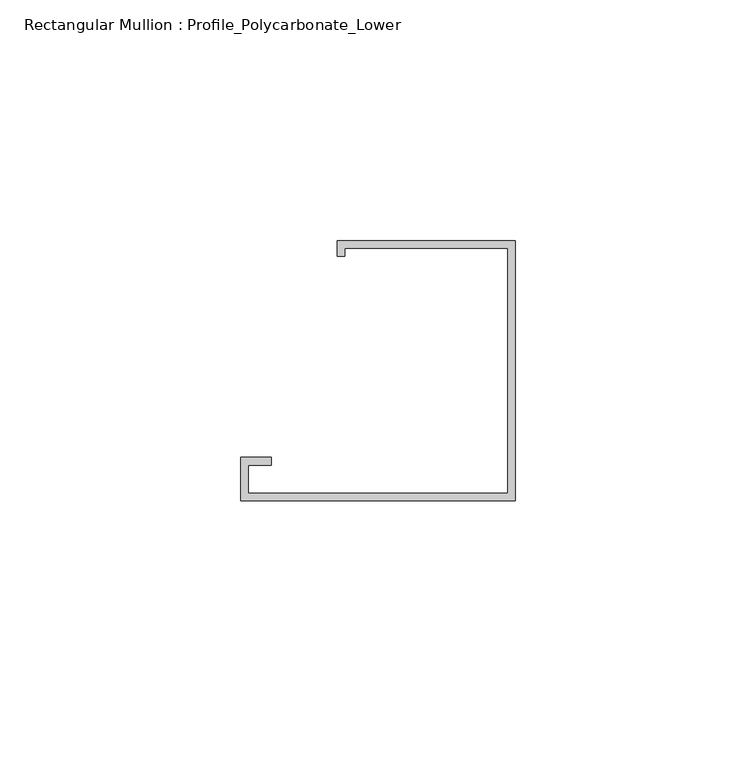
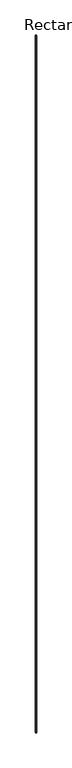
"""IFC4 building model written with IfcOpenShell, lengths in millimetres: member geometry, Rectangular Mullion : Profile_Polycarbonate_Lower."""

import ifcopenshell
import ifcopenshell.guid

model = None  # the IFC model being written
_history = None  # IfcOwnerHistory: only IFC2X3 demands one
_inside = {}  # id of a spatial element -> (the spatial element, [elements in it])
_under = {}  # id of a project, library or spatial element -> (it, [spatial elements below it])
_declared = {}  # id of a project -> (the project, [libraries it declares])
_typed = {}  # id of a type object -> (the type object, [elements of that type])
_made_of = {}  # id of a material, layer set ... -> (it, [elements and type objects made of it])


def new_model(schema):
    """Start an empty IFC model of exactly this schema.

    Asked for "IFC4X3", IfcOpenShell would pick the latest addendum, in which some entities
    have other attributes; the version numbers below select the first issue.
    IFC2X3 requires an IfcOwnerHistory on every rooted entity: one is made here for all.
    """
    global model, _history
    if schema == "IFC4X3":
        model = ifcopenshell.file(schema_version=(4, 3, 0, 0))
    else:
        model = ifcopenshell.file(schema=schema)
    _inside.clear()
    _under.clear()
    _declared.clear()
    _typed.clear()
    _made_of.clear()
    _history = None
    if model.schema == "IFC2X3":
        org = make("IfcOrganization", Name="unknown")
        user = make(
            "IfcPersonAndOrganization",
            ThePerson=make("IfcPerson", FamilyName="unknown"),
            TheOrganization=org,
        )
        app = make(
            "IfcApplication",
            ApplicationDeveloper=org,
            Version="unknown",
            ApplicationFullName="unknown",
            ApplicationIdentifier="unknown",
        )
        _history = make(
            "IfcOwnerHistory",
            OwningUser=user,
            OwningApplication=app,
            ChangeAction="ADDED",
            CreationDate=0,
        )
    return model


def make(cls, **values):
    """One entity of the class cls with the attributes given. An attribute that is None is left unset."""
    return model.create_entity(
        cls, **{name: value for name, value in values.items() if value is not None}
    )


def rooted(cls, **values):
    """An entity with a GlobalId (a new one), such as an element, a storey or a relation."""
    return make(cls, GlobalId=ifcopenshell.guid.new(), OwnerHistory=_history, **values)


def si_unit(unit_type, name, prefix=None):
    """IfcSIUnit, for example si_unit("LENGTHUNIT", "METRE", prefix="MILLI")."""
    return make("IfcSIUnit", UnitType=unit_type, Prefix=prefix, Name=name)


def assignment(units):
    """IfcUnitAssignment: the units of a project."""
    return None if units is None else make("IfcUnitAssignment", Units=units)


def point(xyz):
    """IfcCartesianPoint."""
    return None if xyz is None else make("IfcCartesianPoint", Coordinates=xyz)


def direction(xyz):
    """IfcDirection."""
    return None if xyz is None else make("IfcDirection", DirectionRatios=xyz)


def frame(location, z_axis=None, x_axis=None):
    """IfcAxis2Placement3D, a coordinate frame: its origin and axes. An axis left out is left unset."""
    return make(
        "IfcAxis2Placement3D",
        Location=point(location),
        Axis=direction(z_axis),
        RefDirection=direction(x_axis),
    )


def origin():
    """The frame at (0, 0, 0) with its axes left unset."""
    return frame((0.0, 0.0, 0.0))


def place(relative_to, where):
    """IfcLocalPlacement: puts the frame where relative to a parent placement (None: the world)."""
    return make(
        "IfcLocalPlacement", PlacementRelTo=relative_to, RelativePlacement=where
    )


def context(
    kind, dimensions, precision=None, world=None, true_north=None, identifier=None
):
    """IfcGeometricRepresentationContext, for example the 3D "Model" context."""
    return make(
        "IfcGeometricRepresentationContext",
        ContextIdentifier=identifier,
        ContextType=kind,
        CoordinateSpaceDimension=dimensions,
        Precision=precision,
        WorldCoordinateSystem=world,
        TrueNorth=true_north,
    )


def project(units=None, contexts=None):
    """IfcProject with its units and contexts."""
    return rooted(
        "IfcProject",
        Name="project",
        RepresentationContexts=contexts,
        UnitsInContext=assignment(units),
    )


def spatial(cls, under=None, at=None, **own):
    """A site, building, storey or space (cls), placed at a placement, below another one or the project."""
    s = rooted(cls, ObjectPlacement=at, **own)
    if under is not None:
        _under.setdefault(under.id(), (under, []))[1].append(s)
    return s


def polyline(points):
    """IfcPolyline through the points."""
    return make("IfcPolyline", Points=[point(p) for p in points])


def outline(outer, holes=None, kind="AREA"):
    """IfcArbitraryClosedProfileDef: a profile drawn as a closed curve; with holes, ...WithVoids."""
    if holes is None:
        return make("IfcArbitraryClosedProfileDef", ProfileType=kind, OuterCurve=outer)
    return make(
        "IfcArbitraryProfileDefWithVoids",
        ProfileType=kind,
        OuterCurve=outer,
        InnerCurves=holes,
    )


def extrude(swept, where, along, depth):
    """IfcExtrudedAreaSolid: the profile swept, set in the frame where, extruded along a direction by depth."""
    return make(
        "IfcExtrudedAreaSolid",
        SweptArea=swept,
        Position=where,
        ExtrudedDirection=direction(along),
        Depth=depth,
    )


def shape(context_of_items, identifier, shape_type, items):
    """IfcShapeRepresentation: the items that make up one representation, for example the "Body"."""
    return make(
        "IfcShapeRepresentation",
        ContextOfItems=context_of_items,
        RepresentationIdentifier=identifier,
        RepresentationType=shape_type,
        Items=items,
    )


def source(mapping_origin, context_of_items, identifier, shape_type, items):
    """IfcRepresentationMap: a shape defined once, which mapped items show again and again."""
    return make(
        "IfcRepresentationMap",
        MappingOrigin=mapping_origin,
        MappedRepresentation=shape(context_of_items, identifier, shape_type, items),
    )


def transform(
    local_origin,
    x_axis=None,
    y_axis=None,
    z_axis=None,
    scale=None,
    scale2=None,
    scale3=None,
    uniform=True,
):
    """IfcCartesianTransformationOperator3D, or its non-uniform kind. x_axis, y_axis, z_axis: its Axis1, 2, 3."""
    if uniform:
        return make(
            "IfcCartesianTransformationOperator3D",
            Axis1=direction(x_axis),
            Axis2=direction(y_axis),
            LocalOrigin=point(local_origin),
            Scale=scale,
            Axis3=direction(z_axis),
        )
    return make(
        "IfcCartesianTransformationOperator3DnonUniform",
        Axis1=direction(x_axis),
        Axis2=direction(y_axis),
        LocalOrigin=point(local_origin),
        Scale=scale,
        Axis3=direction(z_axis),
        Scale2=scale2,
        Scale3=scale3,
    )


def mapped(mapping_source, mapping_target):
    """IfcMappedItem: shows the shape of a source again, moved by a transform."""
    return make(
        "IfcMappedItem", MappingSource=mapping_source, MappingTarget=mapping_target
    )


def made_of(thing, what):
    """Note that an element or type object is made of a material, layer set ...; save() writes the relation."""
    if what is not None:
        _made_of.setdefault(what.id(), (what, []))[1].append(thing)
    return thing


def element(
    cls,
    number,
    at=None,
    inside=None,
    cuts=None,
    type_object=None,
    material=None,
    context=None,
    identifier="Body",
    shape_type=None,
    held_by="IfcProductDefinitionShape",
    body=None,
    shapes=None,
    **own,
):
    """One element of the class cls, such as IfcWall. Its Tag is "e" and its number.

    at: its placement. inside: the storey or other place that contains it. cuts: it is an
    opening in that element (IfcRelVoidsElement). A single representation is given by context,
    identifier, shape_type and body (its items); several are given by shapes. held_by: the class
    of the entity that holds the representations. save() writes the other relations.
    """
    e = rooted(cls, Tag="e%d" % number, ObjectPlacement=at, **own)
    if body is not None:
        shapes = [shape(context, identifier, shape_type, body)]
    if shapes is not None:
        e.Representation = make(held_by, Representations=shapes)
    if inside is not None:
        _inside.setdefault(inside.id(), (inside, []))[1].append(e)
    if cuts is not None:
        rooted(
            "IfcRelVoidsElement", RelatingBuildingElement=cuts, RelatedOpeningElement=e
        )
    if type_object is not None:
        _typed.setdefault(type_object.id(), (type_object, []))[1].append(e)
    return made_of(e, material)


def aggregate(whole, parts):
    """IfcRelAggregates: a whole, such as a stair, and the parts it consists of."""
    return rooted("IfcRelAggregates", RelatingObject=whole, RelatedObjects=parts)


def save(model, path):
    """Write the relations noted so far, then the file.

    IfcRelAggregates (storeys below a building ...), IfcRelContainedInSpatialStructure (elements
    in a storey), IfcRelDefinesByType, IfcRelAssociatesMaterial and IfcRelDeclares: one each for
    every whole, place, type object, material and project.
    """
    for whole, parts in _under.values():
        aggregate(whole, parts)
    for where, things in _inside.values():
        rooted(
            "IfcRelContainedInSpatialStructure",
            RelatedElements=things,
            RelatingStructure=where,
        )
    for kind, things in _typed.values():
        rooted("IfcRelDefinesByType", RelatedObjects=things, RelatingType=kind)
    for what, things in _made_of.values():
        rooted("IfcRelAssociatesMaterial", RelatedObjects=things, RelatingMaterial=what)
    for by, libraries in _declared.values():
        rooted("IfcRelDeclares", RelatingContext=by, RelatedDefinitions=libraries)
    model.write(path)


def rectangular_mullion_profile_polycarbonate_lower_2c8e5648(model_context):
    return source(origin(), model_context, "Body", "SweptSolid", [
        extrude(outline(polyline([(0.0, -28.984575), (-56.9976, -28.984575), (-56.9976, -19.992975), (-50.6476, -19.992975), (-50.6476, -21.580475), (-55.4101, -21.580475), (-55.4101, -27.397075), (-1.5875, -27.397075), (-1.5875, 23.428325), (-35.3949, 23.428325), (-35.3949, 21.840825), (-36.9824, 21.840825), (-36.9824, 25.015825), (0.0, 25.015825), (0.0, -28.984575)])), frame((0.0, 0.0, -31532.6903), z_axis=(0.0, 0.0, 1.0), x_axis=(1.0, 0.0, 0.0)), (0.0, 0.0, 1.0), 31532.6903),
    ])


if __name__ == "__main__":
    model = new_model("IFC4")
    model_context = context("Model", 3, world=origin())
    ifc_project = project(units=[si_unit("LENGTHUNIT", "METRE", prefix="MILLI")], contexts=[model_context])
    site = spatial("IfcSite", under=ifc_project)
    building = spatial("IfcBuilding", under=site)
    placement = place(None, origin())
    rectangular_mullion_profile_polycarbonate_lower_shape = rectangular_mullion_profile_polycarbonate_lower_2c8e5648(model_context)
    element("IfcMember", 1, ObjectType="Rectangular Mullion : Profile_Polycarbonate_Lower", at=placement, inside=building, context=model_context, shape_type="MappedRepresentation", body=[
        mapped(rectangular_mullion_profile_polycarbonate_lower_shape, transform((0.0, 0.0, 0.0), x_axis=(1.0, 0.0, 0.0), y_axis=(0.0, 1.0, 0.0), z_axis=(0.0, 0.0, 1.0))),
    ])
    save(model, "model.ifc")

# Revit data of these elements
# Type "Rectangular Mullion : Profile_Polycarbonate_Lower"
#   built-in parameter 1007322 = 0.177167 (stored number, unit not read)
#   built-in parameter 1007321 = 0 (stored number, unit not read)
#   built-in parameter 1007320 = 0.00520833 (stored number, unit not read)
